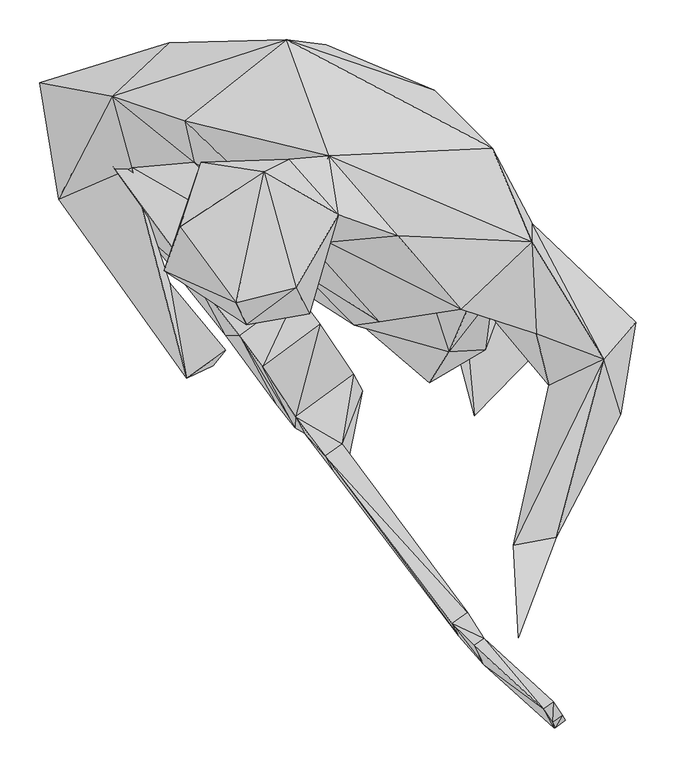
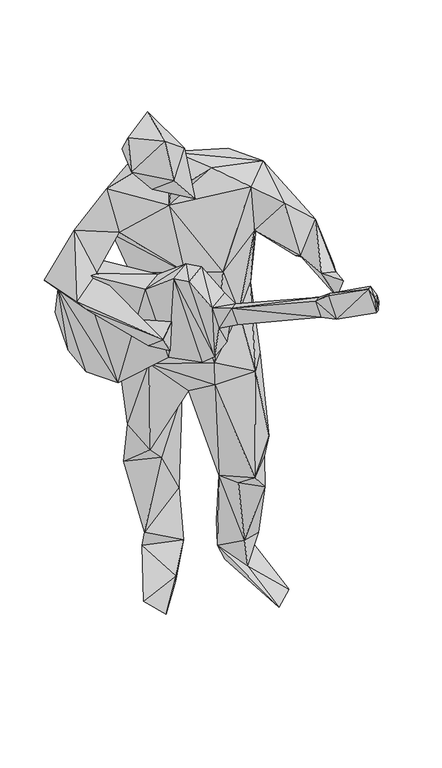
"""IFC4 building model written with IfcOpenShell, lengths in millimetres: geographic element geometry, Enscape AssetDefinition - Andrew 004 Standing : Enscape AssetDefinition - Andrew 004 Standing."""

from ifc_helpers import new_model, si_unit, origin, place, context, project, spatial, faceted_brep, source, transform, mapped, element, save


def geographic_element_775b4b9e(model_context):
    return source(origin(), model_context, "Body", "Brep", [
        faceted_brep([(-401.6925693, -7.7655781, 1045.0603962), (-368.9134419, 74.6408924, 1107.5667143), (-367.7702248, -16.2316673, 1165.5402184), (-289.4049287, -9.7671812, 1277.343154), (-262.3228729, 75.5472556, 1209.5044851), (-320.3763366, 140.1171684, 1236.9214296), (-482.844919, 90.0701135, 1114.782691), (-392.3740685, 73.4327361, 1270.006299), (-173.308, 143.8605636, 1383.0213547), (-123.7316206, 137.6738846, 1180.2920103), (-238.3345962, 13.3806579, 1099.7751951), (-151.3653249, -149.5865583, 1173.6636162), (-168.4823632, 98.9039466, 1013.0857229), (12.0985527, 80.6017295, 1214.2043114), (-81.5260857, 94.8487818, 1016.2084103), (-273.1223106, 13.6144953, 970.3375101), (-247.5541681, -111.7499769, 859.934628), (-199.412778, 99.9762043, 831.39956), (-113.9354557, 123.8815114, 907.5263739), (5.8569112, 67.0971572, 904.8552513), (76.0678947, -3.7363914, 958.4798217), (84.6548975, 8.0094086, 1432.0231676), (134.3571991, -109.007895, 1442.8937435), (134.746924, -86.7304504, 1292.2418118), (-120.2300638, -1.1941663, 1497.389555), (-301.1697531, 42.767141, 1403.1004906), (-459.0325356, -55.8010414, 1118.5090542), (-167.1572924, -86.764425, 1377.4913549), (45.2773906, -193.626821, 1433.2714081), (-56.6204712, -209.5656842, 1177.7867079), (-33.4386528, -101.4641598, 1472.1932411), (-177.636981, -114.5860031, 1440.5251741), (-87.874651, -213.6698216, 869.4710135), (30.3638019, -247.0635027, 817.8260326), (-84.1152743, -208.5464001, 787.9219055), (10.1649035, -186.1400455, 996.2044954), (-109.3206778, -99.6634215, 709.22786), (-41.7708382, -158.423394, 421.4367568), (5.7399925, -286.0542834, 473.7072885), (-212.7974331, -56.99021, 510.6115341), (7.5267451, -122.2056821, 506.642282), (9.1805905, -14.3649708, 744.6721196), (-90.9644887, -31.9936648, 650.6547332), (-239.1250432, 28.5640582, 558.0623746), (-160.8536988, -31.7338444, 451.1899948), (-233.2681417, 60.8175397, 405.9355855), (-83.6176276, 63.4906739, 779.3079019), (-124.9767467, 96.6365337, 502.1594167), (-75.0665963, 14.317004, 285.7784629), (-212.3707384, -23.0808854, 197.2672641), (-124.309212, 89.5444825, 146.7585415), (-255.9403181, 44.6278416, 758.8322163), (-87.7697244, -32.6961726, 133.1140548), (-196.3968724, 17.054094, 122.198686), (-143.1950331, 63.0669668, 18.4741039), (-119.2237586, -43.1878492, 4.6417597), (-151.2723863, -101.3162658, 69.6243942), (-258.4115863, -96.9982818, 15.2663421), (-251.856178, -217.4981534, 40.005073), (67.8166524, -54.0832393, 815.6685233), (84.9397033, -177.072376, 822.8465319), (62.0566756, -125.145629, 553.2767177), (76.3077289, -244.6102202, 572.6102591), (101.1703685, -176.7435968, 452.1813095), (85.5013058, -120.4009429, 1035.7218981), (64.7078305, -180.7188392, 1264.6181583), (-11.7148208, -220.8128273, 422.1872687), (67.6777512, -235.1448387, 389.3651664), (15.495182, -46.7133857, 177.7099371), (-2.2464315, -83.3618045, 114.9067804), (42.2714874, -161.961928, 165.0577635), (104.8707813, -135.3295147, 154.5431018), (47.7526635, -169.9033827, 77.4139538), (87.5698626, -71.7359185, 269.8985636), (109.2127487, -60.6816374, 98.0855227), (59.8891862, -19.6672678, 5.9298598), (142.0458257, -245.8053827, 7.6986253), (62.0376877, -327.080667, 21.9476782), (155.7692587, -288.8133526, 1207.5539827), (179.9433678, -222.5276381, 1158.2913399), (140.323028, -224.4113237, 1358.8613272), (224.4452983, -256.1611533, 1293.7008142), (264.7701502, -210.11132, 1192.0747757), (245.8773404, -325.4787624, 1169.9341536), (165.1486903, -479.4152975, 1263.9086246), (111.0434756, -489.7131026, 1283.3840847), (126.1279434, -551.302135, 1232.9901457), (117.5099611, -605.3274274, 1324.0106106), (-108.4872559, -75.4523277, 1523.2805014), (-258.2836747, -148.0366439, 1503.0195713), (-170.2761203, -5.6520542, 1527.8632641), (-144.6899921, -199.6146441, 1459.8008394), (-326.6469538, -145.4704404, 1584.4957829), (-280.2823186, -9.750193, 1569.9019432), (-223.2041657, -213.2111341, 1560.1707697), (-201.445356, -21.4630142, 1679.1877747), (-306.6649139, -90.6287283, 1667.4349308), (-236.8806303, -185.3705794, 1687.8806353), (-161.6191715, -166.5497273, 1625.2334118), (-319.7797537, -160.6818289, 1071.5119839), (-298.6294925, -280.1284492, 1064.9534464), (-315.7995343, -225.7823646, 1015.8338547), (-249.6227324, -245.2587634, 1089.3354416), (-265.7174766, -264.3784285, 1004.5776367)], [[[0, 1, 2]], [[3, 2, 1]], [[4, 1, 5]], [[6, 1, 0]], [[5, 1, 6]], [[4, 3, 1]], [[7, 5, 6]], [[8, 5, 7]], [[5, 8, 4]], [[4, 9, 10]], [[4, 8, 9]], [[11, 4, 10]], [[11, 3, 4]], [[10, 9, 12]], [[9, 13, 14]], [[14, 12, 9]], [[9, 8, 13]], [[15, 10, 12]], [[10, 15, 16]], [[11, 10, 16]], [[12, 17, 15]], [[12, 18, 17]], [[12, 14, 18]], [[18, 14, 19]], [[14, 20, 19]], [[13, 20, 14]], [[21, 20, 13]], [[8, 21, 13]], [[22, 23, 21]], [[22, 21, 24]], [[24, 21, 8]], [[21, 23, 20]], [[8, 7, 25]], [[25, 24, 8]], [[6, 26, 7]], [[25, 7, 3]], [[7, 26, 2]], [[3, 7, 2]], [[27, 25, 3]], [[27, 24, 25]], [[27, 3, 11]], [[28, 27, 29]], [[30, 27, 28]], [[29, 27, 11]], [[27, 31, 24]], [[30, 31, 27]], [[29, 11, 32]], [[32, 11, 16]], [[33, 32, 34]], [[32, 16, 34]], [[29, 32, 35]], [[33, 35, 32]], [[36, 37, 34]], [[34, 37, 38]], [[34, 38, 33]], [[34, 16, 36]], [[36, 16, 39]], [[36, 40, 37]], [[40, 36, 41]], [[42, 41, 36]], [[42, 36, 39]], [[39, 16, 43]], [[42, 39, 44]], [[39, 43, 45]], [[44, 39, 45]], [[41, 42, 46]], [[47, 42, 48]], [[46, 42, 47]], [[42, 44, 48]], [[45, 49, 44]], [[48, 44, 49]], [[50, 49, 45]], [[47, 50, 45]], [[45, 43, 47]], [[16, 51, 43]], [[43, 51, 47]], [[51, 46, 47]], [[47, 48, 50]], [[50, 48, 52]], [[52, 48, 49]], [[50, 53, 49]], [[52, 49, 53]], [[53, 50, 54]], [[52, 55, 50]], [[54, 50, 55]], [[52, 53, 56]], [[52, 56, 55]], [[53, 54, 57]], [[57, 56, 53]], [[57, 54, 55]], [[58, 57, 55]], [[55, 56, 58]], [[56, 57, 58]], [[51, 15, 17]], [[51, 17, 46]], [[15, 51, 16]], [[18, 46, 17]], [[19, 46, 18]], [[46, 59, 41]], [[46, 19, 59]], [[20, 59, 19]], [[59, 60, 61]], [[41, 59, 61]], [[20, 60, 59]], [[40, 41, 61]], [[62, 63, 61]], [[61, 63, 40]], [[61, 60, 62]], [[64, 33, 60]], [[60, 33, 62]], [[20, 64, 60]], [[20, 23, 64]], [[35, 33, 64]], [[65, 35, 64]], [[65, 64, 23]], [[33, 38, 62]], [[63, 62, 38]], [[38, 37, 66]], [[38, 66, 67]], [[38, 67, 63]], [[37, 68, 69]], [[40, 68, 37]], [[37, 70, 66]], [[37, 69, 70]], [[67, 66, 70]], [[67, 70, 71]], [[63, 67, 71]], [[70, 72, 71]], [[72, 70, 69]], [[73, 71, 74]], [[74, 71, 72]], [[73, 63, 71]], [[40, 63, 73]], [[40, 73, 68]], [[73, 74, 68]], [[69, 68, 74]], [[74, 75, 69]], [[74, 76, 75]], [[74, 72, 76]], [[72, 69, 77]], [[77, 76, 72]], [[77, 75, 76]], [[77, 69, 75]], [[65, 28, 29]], [[78, 65, 79]], [[79, 65, 23]], [[80, 28, 65]], [[35, 65, 29]], [[78, 80, 65]], [[28, 22, 30]], [[28, 80, 22]], [[81, 80, 78]], [[80, 81, 22]], [[22, 24, 30]], [[23, 22, 81]], [[23, 81, 82]], [[82, 79, 23]], [[81, 83, 82]], [[81, 84, 83]], [[81, 78, 85]], [[85, 84, 81]], [[83, 79, 82]], [[86, 78, 83]], [[78, 79, 83]], [[83, 84, 86]], [[87, 86, 84]], [[87, 84, 85]], [[85, 86, 87]], [[85, 78, 86]], [[30, 24, 88]], [[88, 31, 30]], [[31, 89, 90]], [[31, 90, 24]], [[89, 31, 91]], [[88, 91, 31]], [[92, 93, 89]], [[92, 89, 94]], [[94, 89, 91]], [[90, 89, 93]], [[95, 90, 93]], [[90, 88, 24]], [[95, 88, 90]], [[96, 93, 92]], [[95, 93, 96]], [[97, 92, 94]], [[97, 96, 92]], [[94, 91, 98]], [[98, 97, 94]], [[88, 98, 91]], [[98, 95, 97]], [[98, 88, 95]], [[97, 95, 96]], [[2, 99, 0]], [[100, 2, 26]], [[100, 99, 2]], [[101, 100, 0]], [[101, 0, 99]], [[26, 6, 0]], [[0, 100, 26]], [[102, 99, 100]], [[103, 102, 100]], [[100, 101, 103]], [[103, 101, 99]], [[102, 103, 99]]]),
        faceted_brep([(-286.8587375, -157.4530751, 1165.3773785), (-249.532789, -226.5947908, 953.4153342), (-232.4906886, -226.716727, 1224.4061232), (-176.9404709, -173.4848768, 948.8745332), (-186.8475527, -311.2656772, 965.21312), (-346.906811, -104.638949, 823.1313229), (-274.3154764, -51.5290238, 818.5905218), (-162.5355333, -342.0292139, 994.0669537), (-114.256233, -258.1557631, 960.6722593), (-89.9432078, -288.9202833, 989.5261526), (-150.9815902, -349.1602242, 1095.3702927), (-203.6778033, -265.8194304, 1227.6978493), (-162.1058285, -328.5546005, 1158.5401297), (-89.513503, -275.4446864, 1153.9993286), (-104.0163785, -362.1741533, 1173.6536026), (-131.0854703, -212.7095014, 1223.156929), (-125.161618, -377.6453435, 1174.9767065), (-159.899354, -173.6077964, 1219.8653221), (-214.2664045, -104.3431461, 1160.8364582), (-334.3545496, 59.6873276, 1159.5383883), (-406.9468975, 6.5784073, 1164.0791893), (-452.1703124, 62.183585, 1091.4820433), (-379.5790076, 115.2935028, 1086.941123), (-333.9348435, 30.744534, 827.7480602), (-406.5271914, -22.3643854, 832.2889209), (-438.8386309, 26.7992895, 890.7491565), (-387.0607913, 118.4632927, 1004.401803), (-459.652096, 65.3533712, 1008.9435577), (-366.2472963, 79.9082071, 886.2082958), (-78.3892721, -296.0513234, 1090.8293724), (-94.7758332, -379.2922199, 1121.1792231), (-115.9210727, -394.7623968, 1122.502327), (62.2695275, -589.6403193, 1218.9679146), (53.4986518, -573.3937025, 1268.7741518), (43.0509448, -603.7005186, 1220.1701403), (34.2800692, -587.4538422, 1269.9763775), (86.8553594, -630.0401092, 1223.1041193), (73.9443749, -606.123805, 1296.4237928), (74.4330287, -639.1298175, 1223.8805294), (61.5210459, -615.2125001, 1297.201395), (161.8939787, -718.6392546, 1265.2186155), (161.5512073, -685.5253577, 1337.7519846), (174.4631976, -709.4426751, 1264.4323111), (148.9819884, -694.7219968, 1338.5385275), (176.1270314, -709.1099024, 1294.9328423), (160.0332707, -711.7781043, 1315.7323599), (163.5578126, -718.3054686, 1295.7193851), (172.603488, -702.5815248, 1314.9459362)], [[[0, 1, 2]], [[1, 3, 4]], [[5, 6, 1]], [[2, 1, 4]], [[1, 6, 3]], [[0, 5, 1]], [[4, 7, 2]], [[8, 9, 4]], [[4, 3, 8]], [[4, 9, 7]], [[7, 9, 10]], [[11, 7, 12]], [[12, 7, 10]], [[2, 7, 11]], [[13, 12, 14]], [[11, 12, 15]], [[12, 10, 16]], [[14, 12, 16]], [[15, 12, 13]], [[2, 11, 17]], [[17, 11, 15]], [[15, 13, 9]], [[17, 15, 8]], [[8, 15, 9]], [[8, 3, 17]], [[2, 17, 0]], [[17, 3, 18]], [[0, 17, 18]], [[6, 19, 3]], [[3, 19, 18]], [[0, 18, 20]], [[20, 18, 19]], [[20, 5, 0]], [[21, 20, 22]], [[22, 20, 19]], [[21, 5, 20]], [[6, 22, 19]], [[23, 22, 6]], [[5, 23, 6]], [[24, 23, 5]], [[24, 5, 21]], [[24, 21, 25]], [[22, 26, 21]], [[25, 21, 27]], [[21, 26, 27]], [[23, 28, 22]], [[22, 28, 26]], [[24, 25, 23]], [[23, 25, 28]], [[27, 26, 25]], [[25, 26, 28]], [[10, 9, 29]], [[9, 13, 29]], [[29, 30, 10]], [[13, 14, 29]], [[29, 14, 30]], [[16, 10, 31]], [[10, 30, 31]], [[30, 32, 31]], [[14, 33, 30]], [[30, 33, 32]], [[14, 16, 33]], [[31, 34, 16]], [[16, 34, 35]], [[33, 16, 35]], [[31, 32, 34]], [[32, 36, 34]], [[33, 37, 32]], [[32, 37, 36]], [[33, 35, 37]], [[34, 38, 35]], [[37, 35, 39]], [[35, 38, 39]], [[34, 36, 38]], [[38, 36, 40]], [[37, 41, 36]], [[40, 36, 42]], [[36, 41, 42]], [[39, 43, 37]], [[37, 43, 41]], [[39, 38, 43]], [[43, 38, 40]], [[42, 44, 40]], [[43, 40, 45]], [[40, 44, 46]], [[45, 40, 46]], [[41, 47, 42]], [[42, 47, 44]], [[43, 45, 41]], [[41, 45, 47]], [[45, 46, 47]], [[47, 46, 44]]]),
    ])


if __name__ == "__main__":
    model = new_model("IFC4")
    model_context = context("Model", 3, world=origin())
    ifc_project = project(units=[si_unit("LENGTHUNIT", "METRE", prefix="MILLI")], contexts=[model_context])
    site = spatial("IfcSite", under=ifc_project)
    building = spatial("IfcBuilding", under=site)
    placement = place(None, origin())
    geographic_element_shape = geographic_element_775b4b9e(model_context)
    element("IfcGeographicElement", 1, ObjectType="Enscape AssetDefinition - Andrew 004 Standing : Enscape AssetDefinition - Andrew 004 Standing", at=placement, inside=building, context=model_context, shape_type="MappedRepresentation", body=[
        mapped(geographic_element_shape, transform((0.0, 0.0, 0.0), x_axis=(1.0, 0.0, 0.0), y_axis=(0.0, 1.0, 0.0), z_axis=(0.0, 0.0, 1.0))),
    ])
    save(model, "model.ifc")

# Revit data of these elements
# Type "Enscape AssetDefinition - Andrew 004 Standing : Enscape AssetDefinition - Andrew 004 Standing"
#   EnscapeAssetSource = "REMOTE"
#   EnscapeAssetId = "b4e4d0d2-8391-457d-846b-8b8c8d771a96"
#   Height = 1687.881 mm
#   EnscapeNativeAssetHeight = 1687.881 mm
#   Default Elevation = 0
